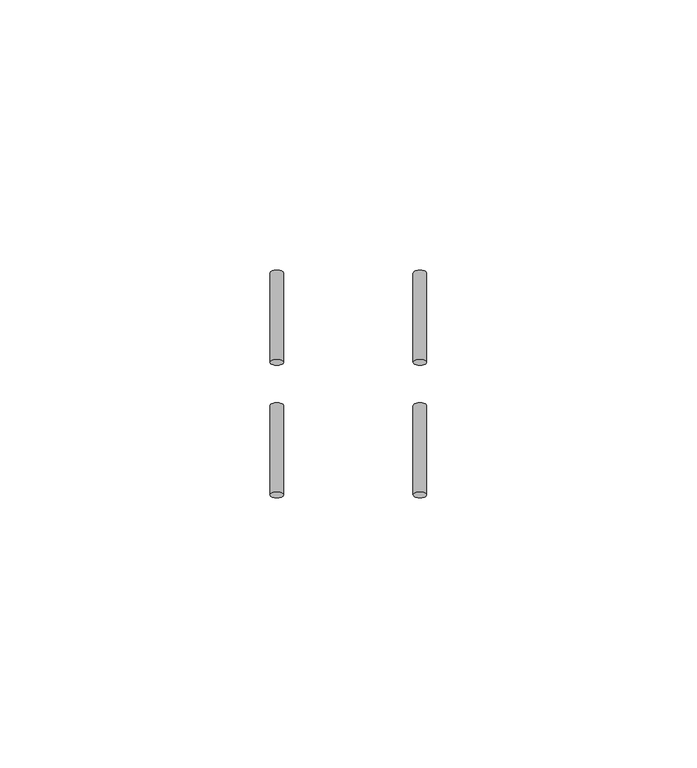
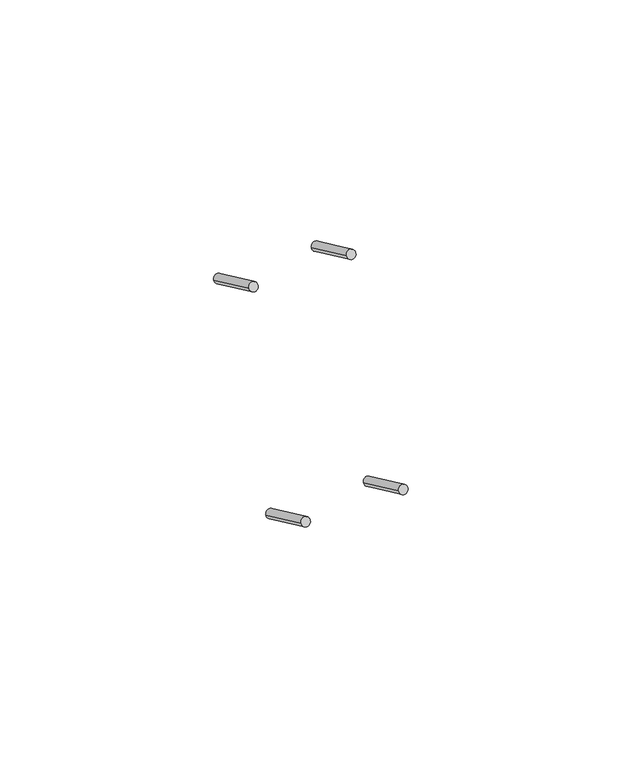
"""IFC4 building model written with IfcOpenShell, lengths in millimetres: furniture geometry, MOLDURA TELA2 : MOLDURA TELA."""

from ifc_helpers import new_model, si_unit, point, frame, frame_2d, origin, place, context, project, spatial, circle_curve, trimmed, segment, composite_curve, outline, extrude, source, transform, mapped, element, save


def furniture_6f4f2263(model_context):
    return source(origin(), model_context, "Body", "SweptSolid", [
        extrude(outline(composite_curve([segment(trimmed(circle_curve(frame_2d((0.0, -1.25)), 1.25), [point((0.0, 0.0))], [point((0.0, -2.5))], False, "CARTESIAN"), True, "CONTINUOUS"), segment(trimmed(circle_curve(frame_2d((0.0, -1.25)), 1.25), [point((0.0, -2.5))], [point((0.0, 0.0))], False, "CARTESIAN"), True, "CONTINUOUS")], self_intersect=False)), frame((2402.7219295, 1333.1379685, 54.4576905), z_axis=(0.0, -0.9063077870366535, 0.4226182617406919), x_axis=(0.0, 0.4226182617406919, 0.9063077870366535)), (0.0, 0.0, 1.0), 18.2226949),
        extrude(outline(composite_curve([segment(trimmed(circle_curve(frame_2d((-58.0000001, -1.25)), 1.25), [point((-58.0000001, -2.5))], [point((-58.0000001, 0.0))], False, "CARTESIAN"), True, "CONTINUOUS"), segment(trimmed(circle_curve(frame_2d((-58.0000001, -1.25)), 1.25), [point((-58.0000001, 0.0))], [point((-58.0000001, -2.5))], False, "CARTESIAN"), True, "CONTINUOUS")], self_intersect=False)), frame((2402.7219295, 1333.1379685, 54.4576905), z_axis=(0.0, -0.9063077870366535, 0.4226182617406919), x_axis=(0.0, 0.4226182617406919, 0.9063077870366535)), (0.0, 0.0, 1.0), 18.2226949),
        extrude(outline(composite_curve([segment(trimmed(circle_curve(frame_2d((-58.0000001, 25.25)), 1.25), [point((-58.0000001, 24.0))], [point((-58.0000001, 26.5))], False, "CARTESIAN"), True, "CONTINUOUS"), segment(trimmed(circle_curve(frame_2d((-58.0000001, 25.25)), 1.25), [point((-58.0000001, 26.5))], [point((-58.0000001, 24.0))], False, "CARTESIAN"), True, "CONTINUOUS")], self_intersect=False)), frame((2402.7219295, 1333.1379685, 54.4576905), z_axis=(0.0, -0.9063077870366535, 0.4226182617406919), x_axis=(0.0, 0.4226182617406919, 0.9063077870366535)), (0.0, 0.0, 1.0), 18.2226949),
        extrude(outline(composite_curve([segment(trimmed(circle_curve(frame_2d((0.0, 25.25)), 1.25), [point((0.0, 24.0))], [point((0.0, 26.5))], False, "CARTESIAN"), True, "CONTINUOUS"), segment(trimmed(circle_curve(frame_2d((0.0, 25.25)), 1.25), [point((0.0, 26.5))], [point((0.0, 24.0))], False, "CARTESIAN"), True, "CONTINUOUS")], self_intersect=False)), frame((2402.7219295, 1333.1379685, 54.4576905), z_axis=(0.0, -0.9063077870366535, 0.4226182617406919), x_axis=(0.0, 0.4226182617406919, 0.9063077870366535)), (0.0, 0.0, 1.0), 18.2226949),
    ])


if __name__ == "__main__":
    model = new_model("IFC4")
    model_context = context("Model", 3, world=origin())
    ifc_project = project(units=[si_unit("LENGTHUNIT", "METRE", prefix="MILLI")], contexts=[model_context])
    site = spatial("IfcSite", under=ifc_project)
    building = spatial("IfcBuilding", under=site)
    placement = place(None, origin())
    furniture_shape = furniture_6f4f2263(model_context)
    element("IfcFurniture", 1, ObjectType="MOLDURA TELA2 : MOLDURA TELA", at=placement, inside=building, context=model_context, shape_type="MappedRepresentation", body=[
        mapped(furniture_shape, transform((0.0, 0.0, 0.0), x_axis=(1.0, 0.0, 0.0), y_axis=(0.0, 1.0, 0.0), z_axis=(0.0, 0.0, 1.0))),
    ])
    save(model, "model.ifc")

# Revit data of these elements
# Type "MOLDURA TELA2 : MOLDURA TELA"
#   Height = 0
# Element 1 (IfcFurniture, "MOLDURA TELA2 : MOLDURA TELA")
#   Materials on its faces: "Aço, Carbono"
# Materials
#   "Aço, Carbono": class "Metal", colour RGB 0 0 0, transparency 0, Description = "Aço Carbono", Cost = 0
